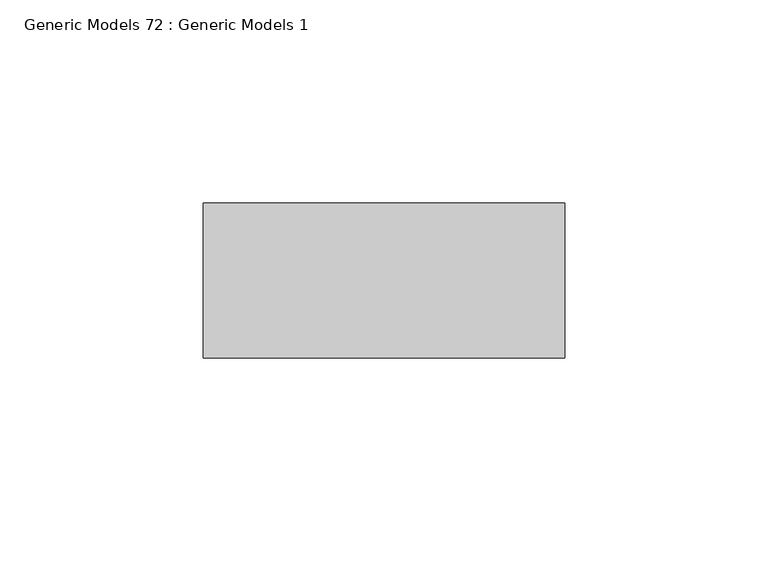
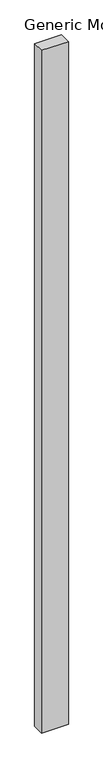
"""IFC4 building model written with IfcOpenShell, lengths in millimetres: proxy geometry, Generic Models 72 : Generic Models 1."""

from ifc_helpers import new_model, si_unit, frame, origin, place, context, project, spatial, polyline, outline, extrude, source, transform, mapped, element, save


def generic_models_72_generic_models_1_f511e09d(model_context):
    return source(origin(), model_context, "Body", "SweptSolid", [
        extrude(outline(polyline([(48561.625, 592.1375), (48472.725, 592.1375), (48472.725, 630.2375), (48561.625, 630.2375), (48561.625, 592.1375)])), frame((0.0, 0.0, 65.950412), z_axis=(0.0, 0.0, 1.0), x_axis=(1.0, 0.0, 0.0)), (0.0, 0.0, 1.0), 2381.25),
    ])


if __name__ == "__main__":
    model = new_model("IFC4")
    model_context = context("Model", 3, world=origin())
    ifc_project = project(units=[si_unit("LENGTHUNIT", "METRE", prefix="MILLI")], contexts=[model_context])
    site = spatial("IfcSite", under=ifc_project)
    building = spatial("IfcBuilding", under=site)
    placement = place(None, origin())
    generic_models_72_generic_models_1_shape = generic_models_72_generic_models_1_f511e09d(model_context)
    element("IfcBuildingElementProxy", 1, Name="Generic Models 72 : Generic Models 1", ObjectType="Generic Models 72 : Generic Models 1", at=placement, inside=building, context=model_context, shape_type="MappedRepresentation", body=[
        mapped(generic_models_72_generic_models_1_shape, transform((0.0, 0.0, 0.0), x_axis=(1.0, 0.0, 0.0), y_axis=(0.0, 1.0, 0.0), z_axis=(0.0, 0.0, 1.0))),
    ])
    save(model, "model.ifc")

# Revit data of these elements
# Element 1 (IfcBuildingElementProxy, "Generic Models 72 : Generic Models 1")
#   Materials on its faces: "METAL STUDS (MATCH EXISTING SIZE/GAUGE/SPACING)"
# Materials
#   "METAL STUDS (MATCH EXISTING SIZE/GAUGE/SPACING)": class "Unassigned", colour RGB 210 209 208, transparency 0, Keynote = "M05121300.02", Cost = 0
